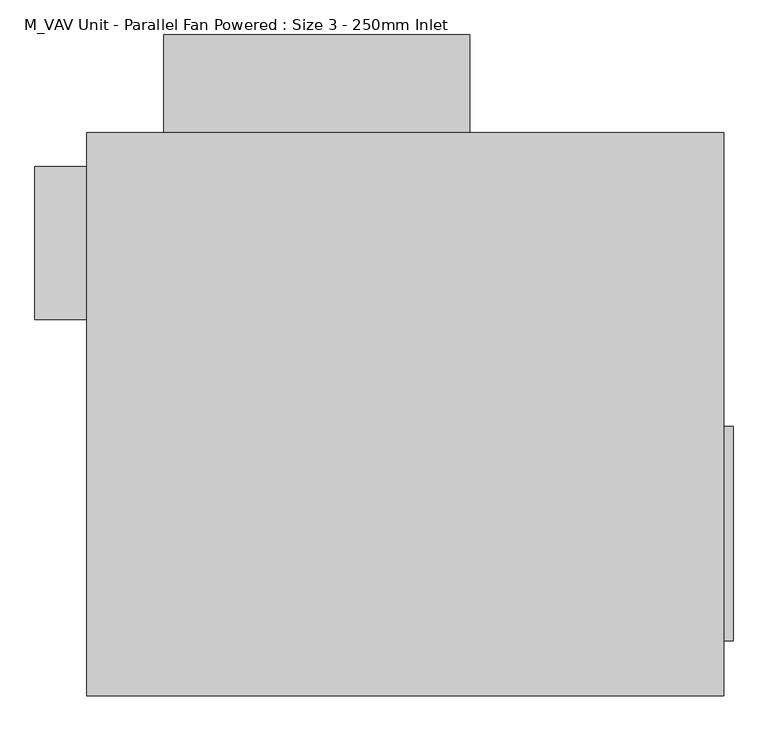
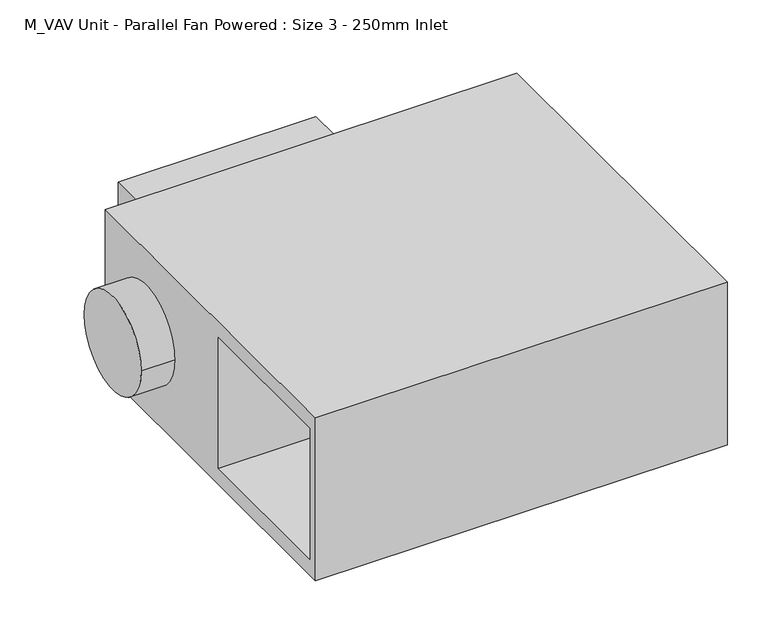
"""IFC4 building model written with IfcOpenShell, lengths in millimetres: proxy geometry, M_VAV Unit - Parallel Fan Powered : Size 3 - 250mm Inlet."""

from ifc_helpers import new_model, si_unit, point, frame, frame_2d, origin, place, context, project, spatial, polyline, circle_curve, trimmed, segment, composite_curve, outline, extrude, faceted_brep, source, transform, mapped, element, save


def m_vav_unit_parallel_fan_powered_size_3_250mm_inlet_cafec42d(model_context):
    return source(origin(), model_context, "Body", "SolidModel", [
        extrude(outline(polyline([(535.0, -20.0), (535.0, -370.0), (519.1125, -370.0), (519.1125, -20.0), (535.0, -20.0)])), frame((0.0, 0.0, -140.0), z_axis=(0.0, 0.0, 1.0), x_axis=(1.0, 0.0, 0.0)), (0.0, 0.0, 1.0), 280.0),
        extrude(outline(polyline([(105.0, 460.0), (-395.0, 460.0), (-395.0, 620.0), (105.0, 620.0), (105.0, 460.0)])), frame((0.0, 0.0, -150.0), z_axis=(0.0, 0.0, 1.0), x_axis=(1.0, 0.0, 0.0)), (0.0, 0.0, 1.0), 300.0),
        extrude(outline(composite_curve([segment(trimmed(circle_curve(frame_2d((280.0, 0.0)), 125.0), [point((155.0, 0.0))], [point((405.0, 0.0))], False, "CARTESIAN"), True, "CONTINUOUS"), segment(trimmed(circle_curve(frame_2d((280.0, 0.0)), 125.0), [point((405.0, 0.0))], [point((155.0, 0.0))], False, "CARTESIAN"), True, "CONTINUOUS")], self_intersect=False)), frame((-605.0, 0.0, 0.0), z_axis=(1.0, 0.0, 0.0), x_axis=(0.0, 1.0, 0.0)), (0.0, 0.0, 1.0), 85.0),
        faceted_brep([(520.0, 460.0, 217.5), (-520.0, 460.0, 217.5), (-520.0, -460.0, 217.5), (520.0, -460.0, 217.5), (520.0, 460.0, -217.5), (520.0, -460.0, -217.5), (-520.0, -460.0, -217.5), (-520.0, 460.0, -217.5), (-520.0, -435.0, 175.0), (-520.0, -435.0, -175.0), (-520.0, -35.0, -175.0), (-520.0, -35.0, 175.0), (0.0, -435.0, 175.0), (0.0, -35.0, 175.0), (0.0, -35.0, -175.0), (0.0, -435.0, -175.0)], [[[0, 1, 2, 3]], [[4, 5, 6, 7]], [[1, 0, 4, 7]], [[2, 1, 7, 6], [8, 9, 10, 11]], [[3, 2, 6, 5]], [[0, 3, 5, 4]], [[12, 13, 14, 15]], [[12, 15, 9, 8]], [[15, 14, 10, 9]], [[14, 13, 11, 10]], [[13, 12, 8, 11]]]),
    ])


if __name__ == "__main__":
    model = new_model("IFC4")
    model_context = context("Model", 3, world=origin())
    ifc_project = project(units=[si_unit("LENGTHUNIT", "METRE", prefix="MILLI")], contexts=[model_context])
    site = spatial("IfcSite", under=ifc_project)
    building = spatial("IfcBuilding", under=site)
    placement = place(None, origin())
    m_vav_unit_parallel_fan_powered_size_3_250mm_inlet_shape = m_vav_unit_parallel_fan_powered_size_3_250mm_inlet_cafec42d(model_context)
    element("IfcBuildingElementProxy", 1, Name="M_VAV Unit - Parallel Fan Powered : Size 3 - 250mm Inlet", ObjectType="M_VAV Unit - Parallel Fan Powered : Size 3 - 250mm Inlet", at=placement, inside=building, context=model_context, shape_type="MappedRepresentation", body=[
        mapped(m_vav_unit_parallel_fan_powered_size_3_250mm_inlet_shape, transform((0.0, 0.0, 0.0), x_axis=(1.0, 0.0, 0.0), y_axis=(0.0, 1.0, 0.0), z_axis=(0.0, 0.0, 1.0))),
    ])
    save(model, "model.ifc")

# Revit data of these elements
# Type "M_VAV Unit - Parallel Fan Powered : Size 3 - 250mm Inlet"
#   Width2 = 350 mm
#   Voltage = 120 V
#   UnitWidth = 1040 mm
#   UnitHeight = 920 mm
#   UnitDepth = 435 mm
#   SupplyConnectorWidth = 350 mm
#   SupplyConnectorVerticalOffset = 54 mm
#   SupplyConnectorLength = 15 mm
#   SupplyConnectorHorizontalOffset = 90 mm
#   SupplyConnectorDepth = 280 mm
#   SupplyAirConnectorCenterOffset = 265 mm
#   PrimaryToSupplyRatio [instance default] = 0.2
#   PrimaryAirOffset = 180 mm
#   PrimaryAirFlow [instance default] = 132.2 L/s
#   PrimaryAirConnectorVerticalOffset = 217.5 mm
#   PrimaryAirConnectorRadius = 125 mm
#   PrimaryAirConnectorLength = 85 mm
#   PrimaryAirConnectorDiameter = 250 mm
#   PrimaryAirConnectorCenterOffset = 180 mm
#   Pressure Drop [instance default] = 2.5 Pa
#   InducedAirInletWidth = 400 mm
#   InducedAirInletDepth = 350 mm
#   InducedAirConnectorHorizontalOffset = 25 mm
#   InducedAirConnectorCenterOffset = 225 mm
#   Height2 = 280 mm
#   ElectricalConnectionBoxWidth = 500 mm
#   ElectricalConnectionBoxOffset = 125 mm
#   ElectricalConnectionBoxHeight = 160 mm
#   ElectricalConnectionBoxDepth = 300 mm
#   SupplyAirFlow [instance default] = 661.0 L/s
#   Apparent Load = 542 VA
#   SupplyAirConnectorIndex = 2
#   PrimaryAirConnectorIndex = 1
#   Number of Poles = 1
#   InducedAirConnectorIndex = 3
#   VAV Material = none
#   Load Classification = Cooling
#   Default Elevation = 0
#   Assembly Code = ""
